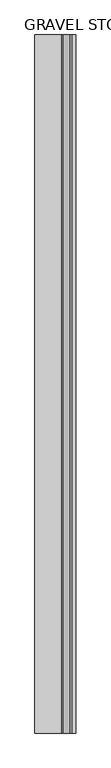
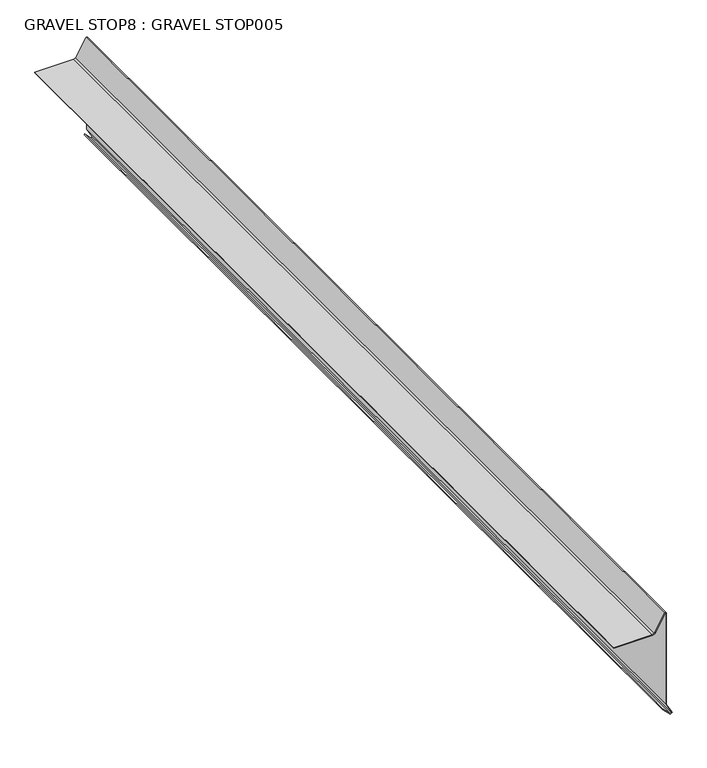
"""IFC4 building model written with IfcOpenShell, lengths in millimetres: proxy geometry, GRAVEL STOP8 : GRAVEL STOP005."""

from ifc_helpers import new_model, si_unit, frame, origin, place, context, project, spatial, polyline, outline, extrude, source, transform, mapped, element, save


def gravel_stop8_gravel_stop005_bb7cdfd3(model_context):
    return source(origin(), model_context, "Body", "SweptSolid", [
        extrude(outline(polyline([(40077.410403, -4353.4420496), (40080.5182783, -4349.3681054), (40101.8558531, -4361.0170744), (40294.5307525, -4361.0170744), (40295.3431515, -4364.0489887), (40259.5408757, -4384.7194423), (40257.3744784, -4388.4717525), (40257.3744784, -4465.9296592), (40255.9633674, -4465.9296592), (40255.9633674, -4388.0936464), (40258.5078708, -4383.6864373), (40293.699878, -4363.3683225), (40293.447969, -4362.4281854), (40101.495749, -4362.4281854), (40080.9054201, -4351.1871656), (40079.2807815, -4353.3168157), (40092.8027062, -4366.8387404), (40091.8049, -4367.8365465), (40077.410403, -4353.4420496)])), frame((0.0, -1065.5906573, 0.0), z_axis=(0.0, 1.0, 0.0), x_axis=(0.0, 0.0, 1.0)), (0.0, 0.0, 1.0), 2000.25),
    ])


if __name__ == "__main__":
    model = new_model("IFC4")
    model_context = context("Model", 3, world=origin())
    ifc_project = project(units=[si_unit("LENGTHUNIT", "METRE", prefix="MILLI")], contexts=[model_context])
    site = spatial("IfcSite", under=ifc_project)
    building = spatial("IfcBuilding", under=site)
    placement = place(None, origin())
    gravel_stop8_gravel_stop005_shape = gravel_stop8_gravel_stop005_bb7cdfd3(model_context)
    element("IfcBuildingElementProxy", 1, Name="GRAVEL STOP8 : GRAVEL STOP005", ObjectType="GRAVEL STOP8 : GRAVEL STOP005", at=placement, inside=building, context=model_context, shape_type="MappedRepresentation", body=[
        mapped(gravel_stop8_gravel_stop005_shape, transform((0.0, 0.0, 0.0), x_axis=(1.0, 0.0, 0.0), y_axis=(0.0, 1.0, 0.0), z_axis=(0.0, 0.0, 1.0))),
    ])
    save(model, "model.ifc")

# Revit data of these elements
# Type "GRAVEL STOP8 : GRAVEL STOP005"
#   NameOverride = "GRAVEL STOP005"
# Element 1 (IfcBuildingElementProxy, "GRAVEL STOP8 : GRAVEL STOP005")
#   Materials on its faces: "GRAVEL STOP REQUIRED WITH GRAVEL SURFACE SYSTEMS"
# Materials
#   "GRAVEL STOP REQUIRED WITH GRAVEL SURFACE SYSTEMS": class "Unassigned", colour RGB 170 170 127, transparency 0, Cost = 0
